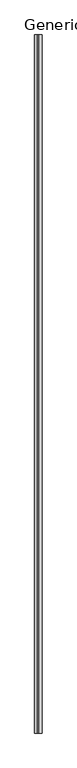
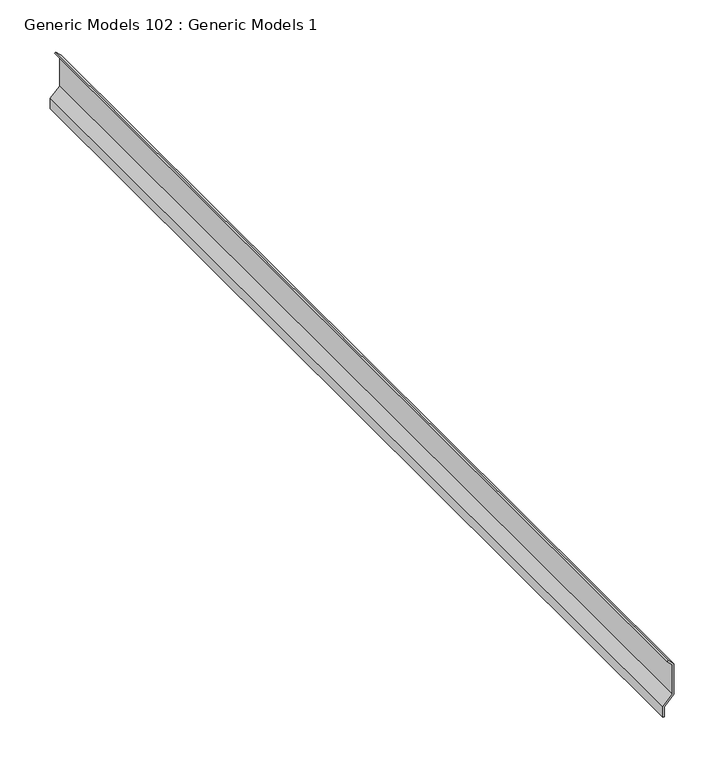
"""IFC4 building model written with IfcOpenShell, lengths in millimetres: proxy geometry, Generic Models 102 : Generic Models 1."""

from ifc_helpers import new_model, si_unit, frame, origin, place, context, project, spatial, polyline, outline, extrude, source, transform, mapped, element, save


def generic_models_102_generic_models_1_1f047596(model_context):
    return source(origin(), model_context, "Body", "SweptSolid", [
        extrude(outline(polyline([(39.3342783, 51003.2), (26.6342783, 51003.2), (26.6342783, 51004.7875), (38.6767142, 51004.7875), (49.7892142, 51015.9), (86.9592783, 51015.9), (93.3092783, 51009.55), (92.1867462, 51008.427468), (86.3017142, 51014.3125), (50.4467783, 51014.3125), (39.3342783, 51003.2)])), frame((0.0, 0.0, 0.0), z_axis=(0.0, 1.0, 0.0), x_axis=(0.0, 0.0, 1.0)), (0.0, 0.0, 1.0), 1219.2),
    ])


if __name__ == "__main__":
    model = new_model("IFC4")
    model_context = context("Model", 3, world=origin())
    ifc_project = project(units=[si_unit("LENGTHUNIT", "METRE", prefix="MILLI")], contexts=[model_context])
    site = spatial("IfcSite", under=ifc_project)
    building = spatial("IfcBuilding", under=site)
    placement = place(None, origin())
    generic_models_102_generic_models_1_shape = generic_models_102_generic_models_1_1f047596(model_context)
    element("IfcBuildingElementProxy", 1, Name="Generic Models 102 : Generic Models 1", ObjectType="Generic Models 102 : Generic Models 1", at=placement, inside=building, context=model_context, shape_type="MappedRepresentation", body=[
        mapped(generic_models_102_generic_models_1_shape, transform((0.0, 0.0, 0.0), x_axis=(1.0, 0.0, 0.0), y_axis=(0.0, 1.0, 0.0), z_axis=(0.0, 0.0, 1.0))),
    ])
    save(model, "model.ifc")

# Revit data of these elements
# Element 1 (IfcBuildingElementProxy, "Generic Models 102 : Generic Models 1")
#   Materials on its faces: "RESILIENT CHANNELS @ 2'-0\""
# Materials
#   "RESILIENT CHANNELS @ 2'-0\"": class "Metal", colour RGB 189 187 185, transparency 0, Description = "Structural steel 50ksi", Cost = 0
